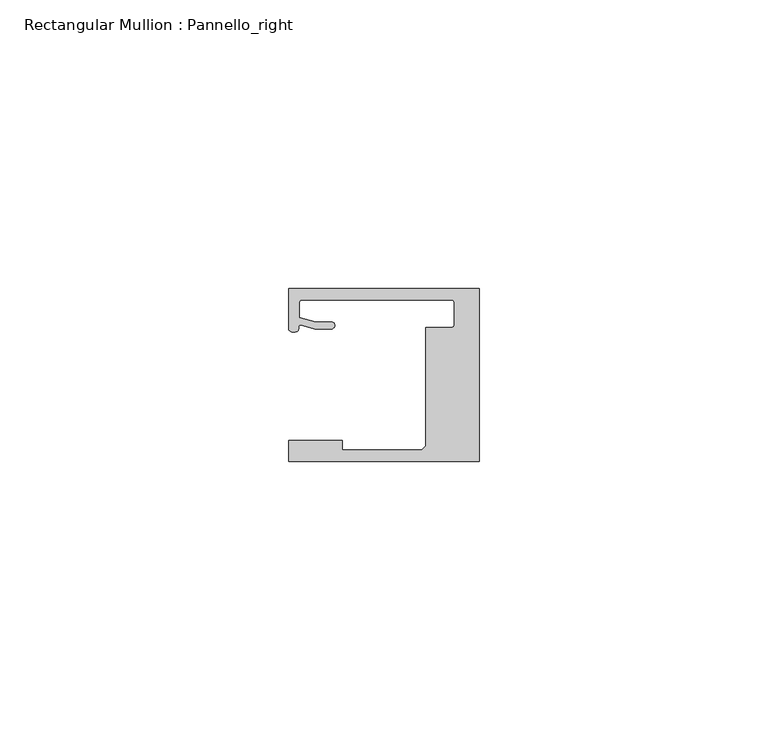
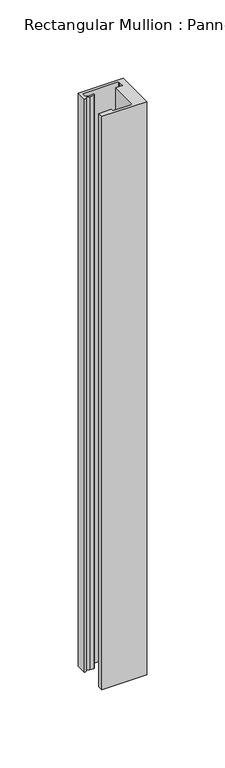
"""IFC4 building model written with IfcOpenShell, lengths in millimetres: member geometry, Rectangular Mullion : Pannello_right."""

import ifcopenshell
import ifcopenshell.guid

model = None  # the IFC model being written
_history = None  # IfcOwnerHistory: only IFC2X3 demands one
_inside = {}  # id of a spatial element -> (the spatial element, [elements in it])
_under = {}  # id of a project, library or spatial element -> (it, [spatial elements below it])
_declared = {}  # id of a project -> (the project, [libraries it declares])
_typed = {}  # id of a type object -> (the type object, [elements of that type])
_made_of = {}  # id of a material, layer set ... -> (it, [elements and type objects made of it])


def new_model(schema):
    """Start an empty IFC model of exactly this schema.

    Asked for "IFC4X3", IfcOpenShell would pick the latest addendum, in which some entities
    have other attributes; the version numbers below select the first issue.
    IFC2X3 requires an IfcOwnerHistory on every rooted entity: one is made here for all.
    """
    global model, _history
    if schema == "IFC4X3":
        model = ifcopenshell.file(schema_version=(4, 3, 0, 0))
    else:
        model = ifcopenshell.file(schema=schema)
    _inside.clear()
    _under.clear()
    _declared.clear()
    _typed.clear()
    _made_of.clear()
    _history = None
    if model.schema == "IFC2X3":
        org = make("IfcOrganization", Name="unknown")
        user = make(
            "IfcPersonAndOrganization",
            ThePerson=make("IfcPerson", FamilyName="unknown"),
            TheOrganization=org,
        )
        app = make(
            "IfcApplication",
            ApplicationDeveloper=org,
            Version="unknown",
            ApplicationFullName="unknown",
            ApplicationIdentifier="unknown",
        )
        _history = make(
            "IfcOwnerHistory",
            OwningUser=user,
            OwningApplication=app,
            ChangeAction="ADDED",
            CreationDate=0,
        )
    return model


def make(cls, **values):
    """One entity of the class cls with the attributes given. An attribute that is None is left unset."""
    return model.create_entity(
        cls, **{name: value for name, value in values.items() if value is not None}
    )


def rooted(cls, **values):
    """An entity with a GlobalId (a new one), such as an element, a storey or a relation."""
    return make(cls, GlobalId=ifcopenshell.guid.new(), OwnerHistory=_history, **values)


def si_unit(unit_type, name, prefix=None):
    """IfcSIUnit, for example si_unit("LENGTHUNIT", "METRE", prefix="MILLI")."""
    return make("IfcSIUnit", UnitType=unit_type, Prefix=prefix, Name=name)


def assignment(units):
    """IfcUnitAssignment: the units of a project."""
    return None if units is None else make("IfcUnitAssignment", Units=units)


def point(xyz):
    """IfcCartesianPoint."""
    return None if xyz is None else make("IfcCartesianPoint", Coordinates=xyz)


def direction(xyz):
    """IfcDirection."""
    return None if xyz is None else make("IfcDirection", DirectionRatios=xyz)


def frame(location, z_axis=None, x_axis=None):
    """IfcAxis2Placement3D, a coordinate frame: its origin and axes. An axis left out is left unset."""
    return make(
        "IfcAxis2Placement3D",
        Location=point(location),
        Axis=direction(z_axis),
        RefDirection=direction(x_axis),
    )


def origin():
    """The frame at (0, 0, 0) with its axes left unset."""
    return frame((0.0, 0.0, 0.0))


def place(relative_to, where):
    """IfcLocalPlacement: puts the frame where relative to a parent placement (None: the world)."""
    return make(
        "IfcLocalPlacement", PlacementRelTo=relative_to, RelativePlacement=where
    )


def context(
    kind, dimensions, precision=None, world=None, true_north=None, identifier=None
):
    """IfcGeometricRepresentationContext, for example the 3D "Model" context."""
    return make(
        "IfcGeometricRepresentationContext",
        ContextIdentifier=identifier,
        ContextType=kind,
        CoordinateSpaceDimension=dimensions,
        Precision=precision,
        WorldCoordinateSystem=world,
        TrueNorth=true_north,
    )


def project(units=None, contexts=None):
    """IfcProject with its units and contexts."""
    return rooted(
        "IfcProject",
        Name="project",
        RepresentationContexts=contexts,
        UnitsInContext=assignment(units),
    )


def spatial(cls, under=None, at=None, **own):
    """A site, building, storey or space (cls), placed at a placement, below another one or the project."""
    s = rooted(cls, ObjectPlacement=at, **own)
    if under is not None:
        _under.setdefault(under.id(), (under, []))[1].append(s)
    return s


def polyline(points):
    """IfcPolyline through the points."""
    return make("IfcPolyline", Points=[point(p) for p in points])


def circle_curve(where, radius):
    """IfcCircle in the frame where."""
    return make("IfcCircle", Position=where, Radius=radius)


def shape(context_of_items, identifier, shape_type, items):
    """IfcShapeRepresentation: the items that make up one representation, for example the "Body"."""
    return make(
        "IfcShapeRepresentation",
        ContextOfItems=context_of_items,
        RepresentationIdentifier=identifier,
        RepresentationType=shape_type,
        Items=items,
    )


def source(mapping_origin, context_of_items, identifier, shape_type, items):
    """IfcRepresentationMap: a shape defined once, which mapped items show again and again."""
    return make(
        "IfcRepresentationMap",
        MappingOrigin=mapping_origin,
        MappedRepresentation=shape(context_of_items, identifier, shape_type, items),
    )


def transform(
    local_origin,
    x_axis=None,
    y_axis=None,
    z_axis=None,
    scale=None,
    scale2=None,
    scale3=None,
    uniform=True,
):
    """IfcCartesianTransformationOperator3D, or its non-uniform kind. x_axis, y_axis, z_axis: its Axis1, 2, 3."""
    if uniform:
        return make(
            "IfcCartesianTransformationOperator3D",
            Axis1=direction(x_axis),
            Axis2=direction(y_axis),
            LocalOrigin=point(local_origin),
            Scale=scale,
            Axis3=direction(z_axis),
        )
    return make(
        "IfcCartesianTransformationOperator3DnonUniform",
        Axis1=direction(x_axis),
        Axis2=direction(y_axis),
        LocalOrigin=point(local_origin),
        Scale=scale,
        Axis3=direction(z_axis),
        Scale2=scale2,
        Scale3=scale3,
    )


def mapped(mapping_source, mapping_target):
    """IfcMappedItem: shows the shape of a source again, moved by a transform."""
    return make(
        "IfcMappedItem", MappingSource=mapping_source, MappingTarget=mapping_target
    )


def made_of(thing, what):
    """Note that an element or type object is made of a material, layer set ...; save() writes the relation."""
    if what is not None:
        _made_of.setdefault(what.id(), (what, []))[1].append(thing)
    return thing


def element(
    cls,
    number,
    at=None,
    inside=None,
    cuts=None,
    type_object=None,
    material=None,
    context=None,
    identifier="Body",
    shape_type=None,
    held_by="IfcProductDefinitionShape",
    body=None,
    shapes=None,
    **own,
):
    """One element of the class cls, such as IfcWall. Its Tag is "e" and its number.

    at: its placement. inside: the storey or other place that contains it. cuts: it is an
    opening in that element (IfcRelVoidsElement). A single representation is given by context,
    identifier, shape_type and body (its items); several are given by shapes. held_by: the class
    of the entity that holds the representations. save() writes the other relations.
    """
    e = rooted(cls, Tag="e%d" % number, ObjectPlacement=at, **own)
    if body is not None:
        shapes = [shape(context, identifier, shape_type, body)]
    if shapes is not None:
        e.Representation = make(held_by, Representations=shapes)
    if inside is not None:
        _inside.setdefault(inside.id(), (inside, []))[1].append(e)
    if cuts is not None:
        rooted(
            "IfcRelVoidsElement", RelatingBuildingElement=cuts, RelatedOpeningElement=e
        )
    if type_object is not None:
        _typed.setdefault(type_object.id(), (type_object, []))[1].append(e)
    return made_of(e, material)


def aggregate(whole, parts):
    """IfcRelAggregates: a whole, such as a stair, and the parts it consists of."""
    return rooted("IfcRelAggregates", RelatingObject=whole, RelatedObjects=parts)


def save(model, path):
    """Write the relations noted so far, then the file.

    IfcRelAggregates (storeys below a building ...), IfcRelContainedInSpatialStructure (elements
    in a storey), IfcRelDefinesByType, IfcRelAssociatesMaterial and IfcRelDeclares: one each for
    every whole, place, type object, material and project.
    """
    for whole, parts in _under.values():
        aggregate(whole, parts)
    for where, things in _inside.values():
        rooted(
            "IfcRelContainedInSpatialStructure",
            RelatedElements=things,
            RelatingStructure=where,
        )
    for kind, things in _typed.values():
        rooted("IfcRelDefinesByType", RelatedObjects=things, RelatingType=kind)
    for what, things in _made_of.values():
        rooted("IfcRelAssociatesMaterial", RelatedObjects=things, RelatingMaterial=what)
    for by, libraries in _declared.values():
        rooted("IfcRelDeclares", RelatingContext=by, RelatedDefinitions=libraries)
    model.write(path)


def plane_surface(at):
    """IfcPlane: the flat surface through the origin of the frame at, square to its z axis."""
    return make("IfcPlane", Position=at)


def cylinder_surface(at, radius):
    """IfcCylindricalSurface: all points at the distance radius from the z axis of the frame at."""
    return make("IfcCylindricalSurface", Position=at, Radius=radius)


def revolved_surface(curve, axis_point, axis_direction):
    """IfcSurfaceOfRevolution: the curve turned about the line through axis_point along axis_direction."""
    return make(
        "IfcSurfaceOfRevolution",
        SweptCurve=make("IfcArbitraryOpenProfileDef", ProfileType="CURVE", Curve=curve),
        AxisPosition=make("IfcAxis1Placement", Location=point(axis_point), Axis=direction(axis_direction)),
    )


def extruded_surface(curve, direction_of_extrusion, depth):
    """IfcSurfaceOfLinearExtrusion: the curve pushed along a direction by depth."""
    return make(
        "IfcSurfaceOfLinearExtrusion",
        SweptCurve=make("IfcArbitraryOpenProfileDef", ProfileType="CURVE", Curve=curve),
        ExtrudedDirection=direction(direction_of_extrusion),
        Depth=depth,
    )


def spline_curve(degree, points, multiplicities, knots, weights=None):
    """IfcBSplineCurveWithKnots; with weights, IfcRationalBSplineCurveWithKnots."""
    own = dict(
        Degree=degree,
        ControlPointsList=[point(p) for p in points],
        CurveForm="UNSPECIFIED",
        ClosedCurve=False,
        SelfIntersect=False,
        KnotMultiplicities=multiplicities,
        Knots=knots,
        KnotSpec="UNSPECIFIED",
    )
    if weights is None:
        return make("IfcBSplineCurveWithKnots", **own)
    return make("IfcRationalBSplineCurveWithKnots", WeightsData=weights, **own)


def advanced_brep(points, edges, surfaces, faces):
    """IfcAdvancedBrep: a solid bounded by faces that lie on surfaces and meet in shared edges.

    An edge is (start, end): straight between two places in points (the first is 0);
    or (start, end, curve); or (start, end, curve, False) where it runs against its curve.
    A face is (place in surfaces, loops), or (place, loops, False) where it looks against
    its surface's normal. A loop lists edges by number (the first is 1), with a minus sign
    where the edge is run from its end to its start. The first loop is the outer one.
    """
    corners = [point(p) for p in points]
    vertices = [make("IfcVertexPoint", VertexGeometry=c) for c in corners]
    made = []
    for start, end, *more in edges:
        made.append(
            make(
                "IfcEdgeCurve",
                EdgeStart=vertices[start],
                EdgeEnd=vertices[end],
                EdgeGeometry=more[0] if more else make("IfcPolyline", Points=[corners[start], corners[end]]),
                SameSense=more[1] if len(more) > 1 else True,
            )
        )
    hull = []
    for where, loops, *sense in faces:
        bounds = []
        for j, loop in enumerate(loops):
            ring = [make("IfcOrientedEdge", EdgeElement=made[abs(k) - 1], Orientation=k > 0) for k in loop]
            bounds.append(
                make(
                    "IfcFaceOuterBound" if j == 0 else "IfcFaceBound",
                    Bound=make("IfcEdgeLoop", EdgeList=ring),
                    Orientation=True,
                )
            )
        hull.append(make("IfcAdvancedFace", Bounds=bounds, FaceSurface=surfaces[where], SameSense=sense[0] if sense else True))
    return make("IfcAdvancedBrep", Outer=make("IfcClosedShell", CfsFaces=hull))


def rectangular_mullion_pannello_right_135688ea(model_context):
    return source(origin(), model_context, "Body", "AdvancedBrep", [
        advanced_brep(
        [(-33.0, -15.0, 0.0), (0.0, -15.0, 0.0), (0.0, 15.0, 0.0), (-33.0000135, 15.0, 0.0), (-33.0000135, 8.0000472, 0.0), (-30.9223017, 8.6490241, 0.0), (-28.4999305, 7.9999523, 0.0), (-25.59998, 7.9999523, 0.0), (-25.59998, 9.1999523, 0.0), (-28.3419477, 9.1999523, 0.0), (-31.19998, 9.9657591, 0.0), (-31.19998, 12.50001, 0.0), (-30.69998, 13.00001, 0.0), (-4.7999726, 13.00001, 0.0), (-4.2999726, 12.50001, 0.0), (-4.2999726, 8.7500595, 0.0), (-4.7999726, 8.2500595, 0.0), (-9.2999726, 8.2500595, 0.0), (-9.2999726, -12.2999849, 0.0), (-10.0000103, -13.0000004, 0.0), (-23.700041, -13.0000004, 0.0), (-23.700041, -11.3000004, 0.0), (-33.0, -11.3000004, 0.0), (-33.0, -15.0, -446.9999865), (-33.0, -11.3000004, -446.9999865), (-23.700041, -11.3000004, -446.9999865), (-23.700041, -13.0000004, -446.9999865), (-10.0000103, -13.0000004, -446.9999865), (-9.2999726, -12.2999849, -446.9999865), (-9.2999726, 8.2500595, -446.9999865), (-4.7999726, 8.2500595, -446.9999865), (-4.2999726, 8.7500595, -446.9999865), (-4.2999726, 12.50001, -446.9999865), (-4.7999726, 13.00001, -446.9999865), (-30.69998, 13.00001, -446.9999865), (-31.19998, 12.50001, -446.9999865), (-31.19998, 9.9657591, -446.9999865), (-28.3419477, 9.1999523, -446.9999865), (-25.59998, 9.1999523, -446.9999865), (-25.59998, 7.9999523, -446.9999865), (-28.4999305, 7.9999523, -446.9999865), (-30.9223017, 8.6490241, -446.9999865), (-33.0000135, 8.0000472, -446.9999865), (-33.0000135, 15.0, -446.9999865), (0.0, 15.0, -446.9999865), (0.0, -15.0, -446.9999865)],
        [
            (0, 1),
            (1, 2),
            (2, 3),
            (3, 4),
            (4, 5, spline_curve(3, [(-33.0000135, 8.0000472, 0.0), (-33.0000135, 7.457047519, 0.0), (-32.262327879, 7.456527435, 0.0), (-31.357433266, 7.563996614, 0.0), (-31.305645054, 7.690065204, 0.0), (-31.298563602, 8.366228555, 0.0), (-31.312054066, 8.717747958, 0.0), (-30.9223017, 8.6490241, 0.0)], [4, 2, 2, 4], [0.0, 0.0027053965905959043, 0.0058611956533709, 0.007702013405570312])),
            (5, 6),
            (6, 7),
            (7, 8, circle_curve(frame((-25.59998, 8.5999523, 0.0), z_axis=(0.0, 0.0, 1.0), x_axis=(0.0, 1.0, 0.0)), 0.6)),
            (8, 9),
            (9, 10),
            (10, 11),
            (11, 12, circle_curve(frame((-30.69998, 12.50001, 0.0), z_axis=(0.0, 0.0, -1.0), x_axis=(0.0, 1.0, 0.0)), 0.5)),
            (12, 13),
            (13, 14, circle_curve(frame((-4.7999726, 12.50001, 0.0), z_axis=(0.0, 0.0, -1.0), x_axis=(1.0, 0.0, 0.0)), 0.5)),
            (14, 15),
            (15, 16, circle_curve(frame((-4.7999726, 8.7500595, 0.0), z_axis=(0.0, 0.0, -1.0), x_axis=(0.0, -1.0, 0.0)), 0.5)),
            (16, 17),
            (17, 18),
            (18, 19),
            (19, 20),
            (20, 21),
            (21, 22),
            (22, 0),
            (23, 24),
            (24, 25),
            (25, 26),
            (26, 27),
            (27, 28),
            (28, 29),
            (29, 30),
            (30, 31, circle_curve(frame((-4.7999726, 8.7500595, -446.9999865), z_axis=(0.0, 0.0, 1.0), x_axis=(0.0, -1.0, 0.0)), 0.5)),
            (31, 32),
            (32, 33, circle_curve(frame((-4.7999726, 12.50001, -446.9999865), z_axis=(0.0, 0.0, 1.0), x_axis=(1.0, 0.0, 0.0)), 0.5)),
            (33, 34),
            (34, 35, circle_curve(frame((-30.69998, 12.50001, -446.9999865), z_axis=(0.0, 0.0, 1.0), x_axis=(0.0, 1.0, 0.0)), 0.5)),
            (35, 36),
            (36, 37),
            (37, 38),
            (38, 39, circle_curve(frame((-25.59998, 8.5999523, -446.9999865), z_axis=(0.0, 0.0, -1.0), x_axis=(0.0, 1.0, 0.0)), 0.6)),
            (39, 40),
            (40, 41),
            (41, 42, spline_curve(3, [(-30.9223017, 8.6490241, -446.9999865), (-31.312054066, 8.717747958, -446.9999865), (-31.298563602, 8.366228555, -446.9999865), (-31.305645054, 7.690065204, -446.9999865), (-31.357433266, 7.563996614, -446.9999865), (-32.262327879, 7.456527435, -446.9999865), (-33.0000135, 7.457047519, -446.9999865), (-33.0000135, 8.0000472, -446.9999865)], [4, 2, 2, 4], [0.0, 0.001840817752199412, 0.004996616814974408, 0.007702013405570312])),
            (42, 43),
            (43, 44),
            (44, 45),
            (45, 23),
            (0, 23),
            (45, 1),
            (44, 2),
            (43, 3),
            (42, 4),
            (41, 5),
            (40, 6),
            (39, 7),
            (38, 8),
            (37, 9),
            (36, 10),
            (35, 11),
            (34, 12),
            (33, 13),
            (32, 14),
            (31, 15),
            (30, 16),
            (29, 17),
            (28, 18),
            (27, 19),
            (26, 20),
            (25, 21),
            (24, 22),
        ],
        [
            plane_surface(frame((0.0, -36.2491502, 0.0), z_axis=(0.0, 0.0, 1.0), x_axis=(-1.0, 0.0, 0.0))),
            plane_surface(frame((0.0, -36.2491502, -446.9999865), z_axis=(0.0, 0.0, -1.0), x_axis=(-1.0, 0.0, 0.0))),
            plane_surface(frame((-33.0, -15.0, 0.0), z_axis=(0.0, -1.0, 0.0), x_axis=(0.0, 0.0, -1.0))),
            plane_surface(frame((0.0, -15.0, 0.0), z_axis=(1.0, 0.0, 0.0), x_axis=(0.0, 0.0, -1.0))),
            plane_surface(frame((0.0, 15.0, 0.0), z_axis=(0.0, 1.0, 0.0), x_axis=(0.0, 0.0, -1.0))),
            plane_surface(frame((-33.0000135, 15.0, 0.0), z_axis=(-1.0, 0.0, 0.0), x_axis=(0.0, 0.0, -1.0))),
            extruded_surface(spline_curve(3, [(-33.0000135, 8.0000472, -446.9999865), (-33.0000135, 7.457047519, -446.9999865), (-32.262327879, 7.456527435, -446.9999865), (-31.357433266, 7.563996614, -446.9999865), (-31.305645054, 7.690065204, -446.9999865), (-31.298563602, 8.366228555, -446.9999865), (-31.312054066, 8.717747958, -446.9999865), (-30.9223017, 8.6490241, -446.9999865)], [4, 2, 2, 4], [0.0, 0.0027053965905959043, 0.0058611956533709, 0.007702013405570312]), (0.0, 0.0, 446.9999865), 446.9999865),
            plane_surface(frame((-30.9223017, 8.6490241, 0.0), z_axis=(-0.2588188320019168, -0.965925883389178, 0.0), x_axis=(0.0, 0.0, -1.0))),
            plane_surface(frame((-28.4999305, 7.9999523, 0.0), z_axis=(0.0, -1.0, 0.0), x_axis=(0.0, 0.0, -1.0))),
            cylinder_surface(frame((-25.59998, 8.5999523, 0.0), z_axis=(0.0, 0.0, 1.0), x_axis=(0.0, 1.0, 0.0)), 0.6),
            plane_surface(frame((-25.59998, 9.1999523, 0.0), z_axis=(0.0, 1.0, 0.0), x_axis=(0.0, 0.0, -1.0))),
            plane_surface(frame((-28.3419477, 9.1999523, 0.0), z_axis=(0.2588188320428738, 0.9659258833782035, 0.0), x_axis=(0.0, 0.0, -1.0))),
            plane_surface(frame((-31.19998, 9.9657591, 0.0), z_axis=(1.0, 0.0, 0.0), x_axis=(0.0, 0.0, -1.0))),
            revolved_surface(polyline([(-30.69998, 13.00001, -446.9999865), (-30.69998, 13.00001, 0.0)]), (-30.69998, 12.50001, 0.0), (0.0, 0.0, -1.0)),
            plane_surface(frame((-30.69998, 13.00001, 0.0), z_axis=(0.0, -1.0, 0.0), x_axis=(0.0, 0.0, -1.0))),
            revolved_surface(polyline([(-4.2999726, 12.50001, -446.9999865), (-4.2999726, 12.50001, 0.0)]), (-4.7999726, 12.50001, 0.0), (0.0, 0.0, -1.0)),
            plane_surface(frame((-4.2999726, 12.50001, 0.0), z_axis=(-1.0, 0.0, 0.0), x_axis=(0.0, 0.0, -1.0))),
            revolved_surface(polyline([(-4.7999726, 8.2500595, -446.9999865), (-4.7999726, 8.2500595, 0.0)]), (-4.7999726, 8.7500595, 0.0), (0.0, 0.0, -1.0)),
            plane_surface(frame((-4.7999726, 8.2500595, 0.0), z_axis=(0.0, 1.0, 0.0), x_axis=(0.0, 0.0, -1.0))),
            plane_surface(frame((-9.2999726, 8.2500595, 0.0), z_axis=(-1.0, 0.0, 0.0), x_axis=(0.0, 0.0, -1.0))),
            plane_surface(frame((-9.2999726, -12.2999849, 0.0), z_axis=(-0.7070955486278075, 0.7071180135668587, 0.0), x_axis=(0.0, 0.0, -1.0))),
            plane_surface(frame((-10.0000103, -13.0000004, 0.0), z_axis=(0.0, 1.0, 0.0), x_axis=(0.0, 0.0, -1.0))),
            plane_surface(frame((-23.700041, -13.0000004, 0.0), z_axis=(1.0, 0.0, 0.0), x_axis=(0.0, 0.0, -1.0))),
            plane_surface(frame((-23.700041, -11.3000004, 0.0), z_axis=(0.0, 1.0, 0.0), x_axis=(0.0, 0.0, -1.0))),
            plane_surface(frame((-33.0, -11.3000004, 0.0), z_axis=(-1.0, 0.0, 0.0), x_axis=(0.0, 0.0, -1.0))),
        ],
        [
            (0, [[1, 2, 3, 4, 5, 6, 7, 8, 9, 10, 11, 12, 13, 14, 15, 16, 17, 18, 19, 20, 21, 22, 23]]),
            (1, [[24, 25, 26, 27, 28, 29, 30, 31, 32, 33, 34, 35, 36, 37, 38, 39, 40, 41, 42, 43, 44, 45, 46]]),
            (2, [[-1, 47, -46, 48]]),
            (3, [[-2, -48, -45, 49]]),
            (4, [[-3, -49, -44, 50]]),
            (5, [[-4, -50, -43, 51]]),
            (6, [[-5, -51, -42, 52]]),
            (7, [[-6, -52, -41, 53]]),
            (8, [[-7, -53, -40, 54]]),
            (9, [[-8, -54, -39, 55]]),
            (10, [[-9, -55, -38, 56]]),
            (11, [[-10, -56, -37, 57]]),
            (12, [[-11, -57, -36, 58]]),
            (13, [[-12, -58, -35, 59]]),
            (14, [[-13, -59, -34, 60]]),
            (15, [[-14, -60, -33, 61]]),
            (16, [[-15, -61, -32, 62]]),
            (17, [[-16, -62, -31, 63]]),
            (18, [[-17, -63, -30, 64]]),
            (19, [[-18, -64, -29, 65]]),
            (20, [[-19, -65, -28, 66]]),
            (21, [[-20, -66, -27, 67]]),
            (22, [[-21, -67, -26, 68]]),
            (23, [[-22, -68, -25, 69]]),
            (24, [[-23, -69, -24, -47]]),
        ],
    ),
    ])


if __name__ == "__main__":
    model = new_model("IFC4")
    model_context = context("Model", 3, world=origin())
    ifc_project = project(units=[si_unit("LENGTHUNIT", "METRE", prefix="MILLI")], contexts=[model_context])
    site = spatial("IfcSite", under=ifc_project)
    building = spatial("IfcBuilding", under=site)
    placement = place(None, origin())
    rectangular_mullion_pannello_right_shape = rectangular_mullion_pannello_right_135688ea(model_context)
    element("IfcMember", 1, ObjectType="Rectangular Mullion : Pannello_right", at=placement, inside=building, context=model_context, shape_type="MappedRepresentation", body=[
        mapped(rectangular_mullion_pannello_right_shape, transform((0.0, 0.0, 0.0), x_axis=(1.0, 0.0, 0.0), y_axis=(0.0, 1.0, 0.0), z_axis=(0.0, 0.0, 1.0))),
    ])
    save(model, "model.ifc")

# Revit data of these elements
# Type "Rectangular Mullion : Pannello_right"
#   built-in parameter 1007322 = 0.0984252 (stored number, unit not read)
#   built-in parameter 1007321 = 0.0305117 (stored number, unit not read)
#   built-in parameter 1007320 = 0 (stored number, unit not read)
